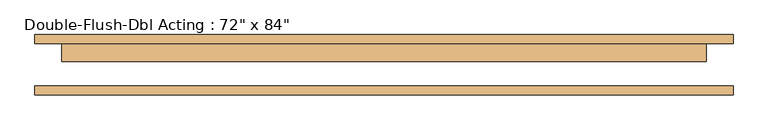
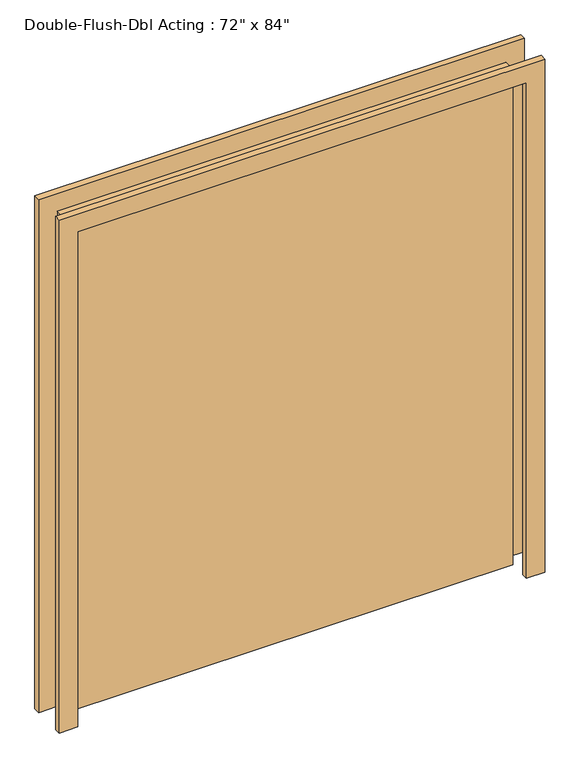
"""IFC4 building model written with IfcOpenShell, lengths in millimetres: door geometry."""

from ifc_helpers import new_model, si_unit, frame, origin, origin_with_axes, place, context, project, spatial, polyline, outline, extrude, source, transform, mapped, element, save


def door_ca526e64(model_context):
    return source(origin(), model_context, "Body", "SweptSolid", [
        extrude(outline(polyline([(2209.8, -990.6), (0.0, -990.6), (0.0, -914.4), (2133.6, -914.4), (2133.6, 914.4), (0.0, 914.4), (0.0, 990.6), (2209.8, 990.6), (2209.8, -990.6)])), frame((0.0, 60.325, 0.0), z_axis=(0.0, 1.0, 0.0), x_axis=(0.0, 0.0, 1.0)), (0.0, 0.0, 1.0), 25.4),
        extrude(outline(polyline([(-914.4, 60.325), (914.4, 60.325), (914.4, 9.525), (-914.4, 9.525), (-914.4, 60.325)])), origin_with_axes(), (0.0, 0.0, 1.0), 2133.6),
        extrude(outline(polyline([(2133.6, -914.4), (2133.6, 914.4), (0.0, 914.4), (0.0, 990.6), (2209.8, 990.6), (2209.8, -990.6), (0.0, -990.6), (0.0, -914.4), (2133.6, -914.4)])), frame((0.0, -85.725, 0.0), z_axis=(0.0, 1.0, 0.0), x_axis=(0.0, 0.0, 1.0)), (0.0, 0.0, 1.0), 25.4),
    ])


if __name__ == "__main__":
    model = new_model("IFC4")
    model_context = context("Model", 3, world=origin())
    ifc_project = project(units=[si_unit("LENGTHUNIT", "METRE", prefix="MILLI")], contexts=[model_context])
    site = spatial("IfcSite", under=ifc_project)
    building = spatial("IfcBuilding", under=site)
    placement = place(None, origin())
    door_shape = door_ca526e64(model_context)
    element("IfcDoor", 1, ObjectType="Double-Flush-Dbl Acting : 72\" x 84\"", at=placement, inside=building, context=model_context, shape_type="MappedRepresentation", body=[
        mapped(door_shape, transform((0.0, 0.0, 0.0), x_axis=(1.0, 0.0, 0.0), y_axis=(0.0, 1.0, 0.0), z_axis=(0.0, 0.0, 1.0))),
    ])
    save(model, "model.ifc")

# Revit data of these elements
# Type "Double-Flush-Dbl Acting : 72\" x 84\""
#   Type Mark = "21"
#   Fire Rating = "20 Min."
#   Assembly Code = "C1020"
#   Thickness = 50.8 mm
#   Height = 2133.6 mm
#   Trim Projection Ext. = 25.4 mm
#   Trim Projection Int. = 25.4 mm
#   Trim Width Ext. = 76.2 mm
#   Trim Width Int. = 76.2 mm
#   Width = 1828.8 mm
#   Define Thermal Properties by = 0
#   Door Material = Door - Panel
#   Frame Material = Door - Frame
#   Function = (empty or 0)
#   Wall Closure = (empty or 0)
# Element 1 (IfcDoor, "Double-Flush-Dbl Acting : 72\" x 84\"")
#   Materials on its faces: "Door - Frame", "Door - Panel"
# Materials
#   "Door - Panel": class "Wood", colour RGB 210 159 95, transparency 0, Cost = 0
#   "Door - Frame": class "Miscellaneous", colour RGB 118 70 51, transparency 0, Cost = 0
